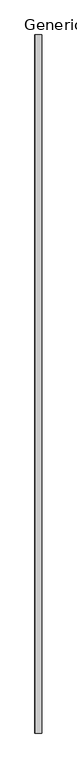
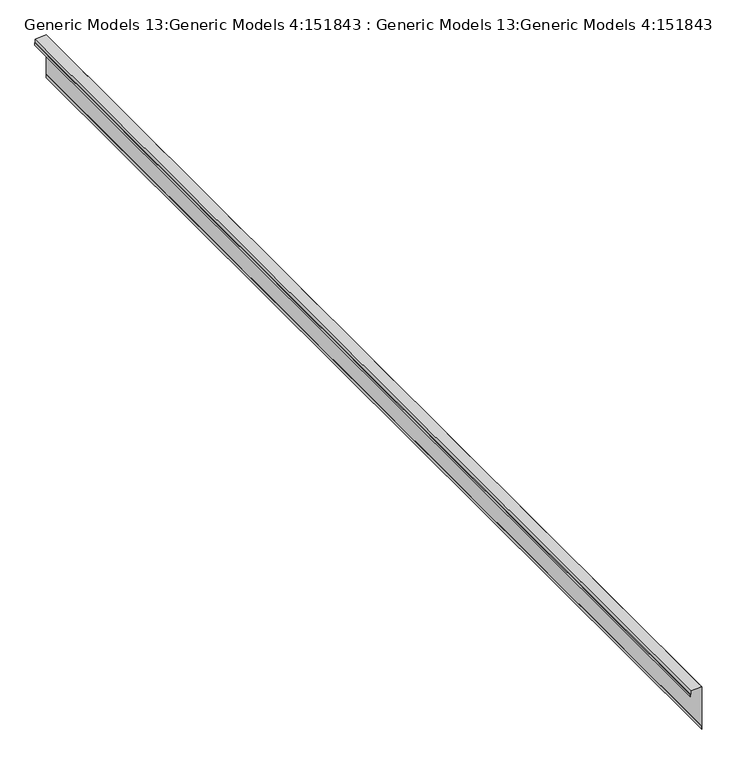
"""IFC4 building model written with IfcOpenShell, lengths in millimetres: proxy geometry, Generic Models 13:Generic Models 4:151843 : Generic Models 13:Generic Models 4:151843."""

from ifc_helpers import new_model, si_unit, frame, origin, place, context, project, spatial, polyline, outline, extrude, source, transform, mapped, element, save


def generic_models_13_generic_models_4_151843_generic_models_13_0d1c5031(model_context):
    return source(origin(), model_context, "Body", "SweptSolid", [
        extrude(outline(polyline([(3676.3784351, 8347.929274), (3715.6290789, 8347.929274), (3722.7610194, 8350.525088), (3780.4680881, 8350.525088), (3788.0478493, 8532.4393587), (3104.036454, 8532.4393587), (3095.123518, 8535.6834021), (3048.1011943, 8535.6834021), (3048.1011943, 8536.4771521), (3095.6243108, 8536.4771521), (3104.5372468, 8533.2331087), (3788.875361, 8533.2331087), (3781.2294539, 8349.731338), (3722.900979, 8349.731338), (3715.7690384, 8347.135524), (3676.3784351, 8347.135524), (3676.3784351, 8347.929274)])), frame((0.0, -6674.7974793, 0.0), z_axis=(0.0, 1.0, 0.0), x_axis=(0.0, 0.0, 1.0)), (0.0, 0.0, 1.0), 18643.6),
    ])


if __name__ == "__main__":
    model = new_model("IFC4")
    model_context = context("Model", 3, world=origin())
    ifc_project = project(units=[si_unit("LENGTHUNIT", "METRE", prefix="MILLI")], contexts=[model_context])
    site = spatial("IfcSite", under=ifc_project)
    building = spatial("IfcBuilding", under=site)
    placement = place(None, origin())
    generic_models_13_generic_models_4_151843_generic_models_13_shape = generic_models_13_generic_models_4_151843_generic_models_13_0d1c5031(model_context)
    element("IfcBuildingElementProxy", 1, Name="Generic Models 13:Generic Models 4:151843 : Generic Models 13:Generic Models 4:151843", ObjectType="Generic Models 13:Generic Models 4:151843 : Generic Models 13:Generic Models 4:151843", at=placement, inside=building, context=model_context, shape_type="MappedRepresentation", body=[
        mapped(generic_models_13_generic_models_4_151843_generic_models_13_shape, transform((0.0, 0.0, 0.0), x_axis=(1.0, 0.0, 0.0), y_axis=(0.0, 1.0, 0.0), z_axis=(0.0, 0.0, 1.0))),
    ])
    save(model, "model.ifc")

# Revit data of these elements
# Type "Generic Models 13:Generic Models 4:151843 : Generic Models 13:Generic Models 4:151843"
#   NameOverride = "Generic Models 13:Generic Models 4:151843"
#   ObjectTypeOverride = "Generic Models 13:Generic Models 4"
#   Reference = "Generic Models 4"
#   Category = "Generic Models"
#   Tag = "151843"
# Element 1 (IfcBuildingElementProxy, "Generic Models 13:Generic Models 4:151843 : Generic Models 13:Generic Models 4:151843")
#   Materials on its faces: "_(2) LAYERS NO. 30 ASTM D226 ASPHALT SATURATED ORGANIC FELT 997"
# Materials
#   "_(2) LAYERS NO. 30 ASTM D226 ASPHALT SATURATED ORGANIC FELT 997": class "Unassigned", colour RGB 67 154 161, transparency 0
